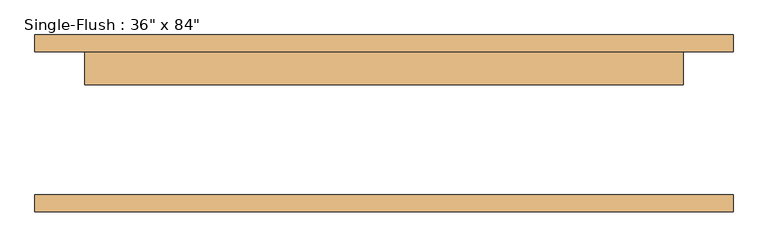
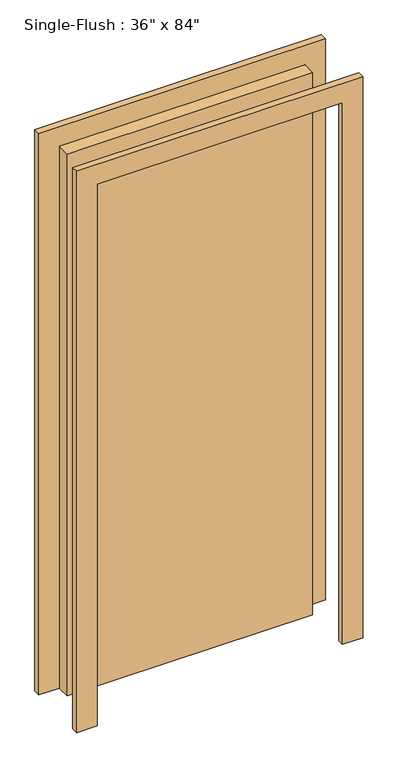
"""IFC4 building model written with IfcOpenShell, lengths in millimetres: door geometry."""

from ifc_helpers import new_model, si_unit, frame, origin, origin_with_axes, place, context, project, spatial, polyline, outline, extrude, source, transform, mapped, element, save


def door_6952d7f5(model_context):
    return source(origin(), model_context, "Body", "SweptSolid", [
        extrude(outline(polyline([(2209.8, -533.4), (0.0, -533.4), (0.0, -457.2), (2133.6, -457.2), (2133.6, 457.2), (0.0, 457.2), (0.0, 533.4), (2209.8, 533.4), (2209.8, -533.4)])), frame((0.0, 109.5375, 0.0), z_axis=(0.0, 1.0, 0.0), x_axis=(0.0, 0.0, 1.0)), (0.0, 0.0, 1.0), 25.4),
        extrude(outline(polyline([(2209.8, 533.4), (2209.8, -533.4), (0.0, -533.4), (0.0, -457.2), (2133.6, -457.2), (2133.6, 457.2), (0.0, 457.2), (0.0, 533.4), (2209.8, 533.4)])), frame((0.0, -134.9375, 0.0), z_axis=(0.0, 1.0, 0.0), x_axis=(0.0, 0.0, 1.0)), (0.0, 0.0, 1.0), 25.4),
        extrude(outline(polyline([(457.2, 58.7375), (-457.2, 58.7375), (-457.2, 109.5375), (457.2, 109.5375), (457.2, 58.7375)])), origin_with_axes(), (0.0, 0.0, 1.0), 2133.6),
    ])


if __name__ == "__main__":
    model = new_model("IFC4")
    model_context = context("Model", 3, world=origin())
    ifc_project = project(units=[si_unit("LENGTHUNIT", "METRE", prefix="MILLI")], contexts=[model_context])
    site = spatial("IfcSite", under=ifc_project)
    building = spatial("IfcBuilding", under=site)
    placement = place(None, origin())
    door_shape = door_6952d7f5(model_context)
    element("IfcDoor", 1, ObjectType="Single-Flush : 36\" x 84\"", at=placement, inside=building, context=model_context, shape_type="MappedRepresentation", body=[
        mapped(door_shape, transform((0.0, 0.0, 0.0), x_axis=(1.0, 0.0, 0.0), y_axis=(0.0, 1.0, 0.0), z_axis=(0.0, 0.0, 1.0))),
    ])
    save(model, "model.ifc")

# Revit data of these elements
# Type "Single-Flush : 36\" x 84\""
#   Type Mark = "1"
#   Assembly Code = "C1020"
#   Thickness = 0' - 2"
#   Height = 7' - 0"
#   Trim Projection Ext = 0' - 1"
#   Trim Projection Int = 0' - 1"
#   Trim Width = 0' - 3"
#   Width = 3' - 0"
#   Door Material = none
#   Frame Material = none
#   Function = (empty or 0)
#   Wall Closure = (empty or 0)
